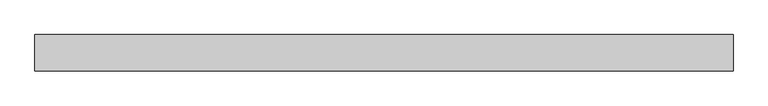
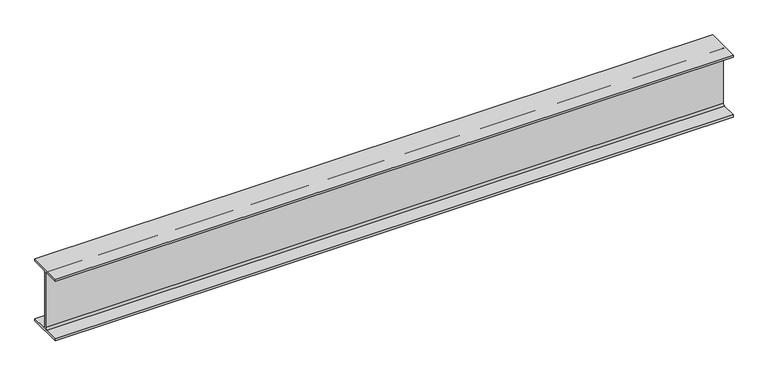
"""IFC4 building model written with IfcOpenShell, lengths in millimetres: beam geometry, Old_Steel Beam_H-KSD3502 : H_SB_ASB_H-250×125x6x9."""

import ifcopenshell
import ifcopenshell.guid

model = None  # the IFC model being written
_history = None  # IfcOwnerHistory: only IFC2X3 demands one
_inside = {}  # id of a spatial element -> (the spatial element, [elements in it])
_under = {}  # id of a project, library or spatial element -> (it, [spatial elements below it])
_declared = {}  # id of a project -> (the project, [libraries it declares])
_typed = {}  # id of a type object -> (the type object, [elements of that type])
_made_of = {}  # id of a material, layer set ... -> (it, [elements and type objects made of it])


def new_model(schema):
    """Start an empty IFC model of exactly this schema.

    Asked for "IFC4X3", IfcOpenShell would pick the latest addendum, in which some entities
    have other attributes; the version numbers below select the first issue.
    IFC2X3 requires an IfcOwnerHistory on every rooted entity: one is made here for all.
    """
    global model, _history
    if schema == "IFC4X3":
        model = ifcopenshell.file(schema_version=(4, 3, 0, 0))
    else:
        model = ifcopenshell.file(schema=schema)
    _inside.clear()
    _under.clear()
    _declared.clear()
    _typed.clear()
    _made_of.clear()
    _history = None
    if model.schema == "IFC2X3":
        org = make("IfcOrganization", Name="unknown")
        user = make(
            "IfcPersonAndOrganization",
            ThePerson=make("IfcPerson", FamilyName="unknown"),
            TheOrganization=org,
        )
        app = make(
            "IfcApplication",
            ApplicationDeveloper=org,
            Version="unknown",
            ApplicationFullName="unknown",
            ApplicationIdentifier="unknown",
        )
        _history = make(
            "IfcOwnerHistory",
            OwningUser=user,
            OwningApplication=app,
            ChangeAction="ADDED",
            CreationDate=0,
        )
    return model


def make(cls, **values):
    """One entity of the class cls with the attributes given. An attribute that is None is left unset."""
    return model.create_entity(
        cls, **{name: value for name, value in values.items() if value is not None}
    )


def rooted(cls, **values):
    """An entity with a GlobalId (a new one), such as an element, a storey or a relation."""
    return make(cls, GlobalId=ifcopenshell.guid.new(), OwnerHistory=_history, **values)


def si_unit(unit_type, name, prefix=None):
    """IfcSIUnit, for example si_unit("LENGTHUNIT", "METRE", prefix="MILLI")."""
    return make("IfcSIUnit", UnitType=unit_type, Prefix=prefix, Name=name)


def assignment(units):
    """IfcUnitAssignment: the units of a project."""
    return None if units is None else make("IfcUnitAssignment", Units=units)


def point(xyz):
    """IfcCartesianPoint."""
    return None if xyz is None else make("IfcCartesianPoint", Coordinates=xyz)


def direction(xyz):
    """IfcDirection."""
    return None if xyz is None else make("IfcDirection", DirectionRatios=xyz)


def frame(location, z_axis=None, x_axis=None):
    """IfcAxis2Placement3D, a coordinate frame: its origin and axes. An axis left out is left unset."""
    return make(
        "IfcAxis2Placement3D",
        Location=point(location),
        Axis=direction(z_axis),
        RefDirection=direction(x_axis),
    )


def frame_2d(location, x_axis=None):
    """IfcAxis2Placement2D, a coordinate frame in the plane: its origin and x axis."""
    return make(
        "IfcAxis2Placement2D", Location=point(location), RefDirection=direction(x_axis)
    )


def origin():
    """The frame at (0, 0, 0) with its axes left unset."""
    return frame((0.0, 0.0, 0.0))


def place(relative_to, where):
    """IfcLocalPlacement: puts the frame where relative to a parent placement (None: the world)."""
    return make(
        "IfcLocalPlacement", PlacementRelTo=relative_to, RelativePlacement=where
    )


def context(
    kind, dimensions, precision=None, world=None, true_north=None, identifier=None
):
    """IfcGeometricRepresentationContext, for example the 3D "Model" context."""
    return make(
        "IfcGeometricRepresentationContext",
        ContextIdentifier=identifier,
        ContextType=kind,
        CoordinateSpaceDimension=dimensions,
        Precision=precision,
        WorldCoordinateSystem=world,
        TrueNorth=true_north,
    )


def project(units=None, contexts=None):
    """IfcProject with its units and contexts."""
    return rooted(
        "IfcProject",
        Name="project",
        RepresentationContexts=contexts,
        UnitsInContext=assignment(units),
    )


def spatial(cls, under=None, at=None, **own):
    """A site, building, storey or space (cls), placed at a placement, below another one or the project."""
    s = rooted(cls, ObjectPlacement=at, **own)
    if under is not None:
        _under.setdefault(under.id(), (under, []))[1].append(s)
    return s


def polyline(points):
    """IfcPolyline through the points."""
    return make("IfcPolyline", Points=[point(p) for p in points])


def circle_curve(where, radius):
    """IfcCircle in the frame where."""
    return make("IfcCircle", Position=where, Radius=radius)


def trimmed(basis, trim1, trim2, sense, master):
    """IfcTrimmedCurve: the piece of a basis curve between two trims."""
    return make(
        "IfcTrimmedCurve",
        BasisCurve=basis,
        Trim1=trim1,
        Trim2=trim2,
        SenseAgreement=sense,
        MasterRepresentation=master,
    )


def segment(curve, same_sense, transition):
    """IfcCompositeCurveSegment."""
    return make(
        "IfcCompositeCurveSegment",
        Transition=transition,
        SameSense=same_sense,
        ParentCurve=curve,
    )


def composite_curve(segments, self_intersect=None):
    """IfcCompositeCurve: segments joined end to end."""
    return make("IfcCompositeCurve", Segments=segments, SelfIntersect=self_intersect)


def outline(outer, holes=None, kind="AREA"):
    """IfcArbitraryClosedProfileDef: a profile drawn as a closed curve; with holes, ...WithVoids."""
    if holes is None:
        return make("IfcArbitraryClosedProfileDef", ProfileType=kind, OuterCurve=outer)
    return make(
        "IfcArbitraryProfileDefWithVoids",
        ProfileType=kind,
        OuterCurve=outer,
        InnerCurves=holes,
    )


def extrude(swept, where, along, depth):
    """IfcExtrudedAreaSolid: the profile swept, set in the frame where, extruded along a direction by depth."""
    return make(
        "IfcExtrudedAreaSolid",
        SweptArea=swept,
        Position=where,
        ExtrudedDirection=direction(along),
        Depth=depth,
    )


def shape(context_of_items, identifier, shape_type, items):
    """IfcShapeRepresentation: the items that make up one representation, for example the "Body"."""
    return make(
        "IfcShapeRepresentation",
        ContextOfItems=context_of_items,
        RepresentationIdentifier=identifier,
        RepresentationType=shape_type,
        Items=items,
    )


def source(mapping_origin, context_of_items, identifier, shape_type, items):
    """IfcRepresentationMap: a shape defined once, which mapped items show again and again."""
    return make(
        "IfcRepresentationMap",
        MappingOrigin=mapping_origin,
        MappedRepresentation=shape(context_of_items, identifier, shape_type, items),
    )


def transform(
    local_origin,
    x_axis=None,
    y_axis=None,
    z_axis=None,
    scale=None,
    scale2=None,
    scale3=None,
    uniform=True,
):
    """IfcCartesianTransformationOperator3D, or its non-uniform kind. x_axis, y_axis, z_axis: its Axis1, 2, 3."""
    if uniform:
        return make(
            "IfcCartesianTransformationOperator3D",
            Axis1=direction(x_axis),
            Axis2=direction(y_axis),
            LocalOrigin=point(local_origin),
            Scale=scale,
            Axis3=direction(z_axis),
        )
    return make(
        "IfcCartesianTransformationOperator3DnonUniform",
        Axis1=direction(x_axis),
        Axis2=direction(y_axis),
        LocalOrigin=point(local_origin),
        Scale=scale,
        Axis3=direction(z_axis),
        Scale2=scale2,
        Scale3=scale3,
    )


def mapped(mapping_source, mapping_target):
    """IfcMappedItem: shows the shape of a source again, moved by a transform."""
    return make(
        "IfcMappedItem", MappingSource=mapping_source, MappingTarget=mapping_target
    )


def made_of(thing, what):
    """Note that an element or type object is made of a material, layer set ...; save() writes the relation."""
    if what is not None:
        _made_of.setdefault(what.id(), (what, []))[1].append(thing)
    return thing


def element(
    cls,
    number,
    at=None,
    inside=None,
    cuts=None,
    type_object=None,
    material=None,
    context=None,
    identifier="Body",
    shape_type=None,
    held_by="IfcProductDefinitionShape",
    body=None,
    shapes=None,
    **own,
):
    """One element of the class cls, such as IfcWall. Its Tag is "e" and its number.

    at: its placement. inside: the storey or other place that contains it. cuts: it is an
    opening in that element (IfcRelVoidsElement). A single representation is given by context,
    identifier, shape_type and body (its items); several are given by shapes. held_by: the class
    of the entity that holds the representations. save() writes the other relations.
    """
    e = rooted(cls, Tag="e%d" % number, ObjectPlacement=at, **own)
    if body is not None:
        shapes = [shape(context, identifier, shape_type, body)]
    if shapes is not None:
        e.Representation = make(held_by, Representations=shapes)
    if inside is not None:
        _inside.setdefault(inside.id(), (inside, []))[1].append(e)
    if cuts is not None:
        rooted(
            "IfcRelVoidsElement", RelatingBuildingElement=cuts, RelatedOpeningElement=e
        )
    if type_object is not None:
        _typed.setdefault(type_object.id(), (type_object, []))[1].append(e)
    return made_of(e, material)


def aggregate(whole, parts):
    """IfcRelAggregates: a whole, such as a stair, and the parts it consists of."""
    return rooted("IfcRelAggregates", RelatingObject=whole, RelatedObjects=parts)


def save(model, path):
    """Write the relations noted so far, then the file.

    IfcRelAggregates (storeys below a building ...), IfcRelContainedInSpatialStructure (elements
    in a storey), IfcRelDefinesByType, IfcRelAssociatesMaterial and IfcRelDeclares: one each for
    every whole, place, type object, material and project.
    """
    for whole, parts in _under.values():
        aggregate(whole, parts)
    for where, things in _inside.values():
        rooted(
            "IfcRelContainedInSpatialStructure",
            RelatedElements=things,
            RelatingStructure=where,
        )
    for kind, things in _typed.values():
        rooted("IfcRelDefinesByType", RelatedObjects=things, RelatingType=kind)
    for what, things in _made_of.values():
        rooted("IfcRelAssociatesMaterial", RelatedObjects=things, RelatingMaterial=what)
    for by, libraries in _declared.values():
        rooted("IfcRelDeclares", RelatingContext=by, RelatedDefinitions=libraries)
    model.write(path)


def beam_56242eb7(model_context):
    return source(origin(), model_context, "Body", "SweptSolid", [
        extrude(outline(composite_curve([segment(polyline([(82.5, -141.5), (82.5, -151.7), (-82.5, -151.7), (-82.5, -141.5), (-11.9, -141.5)]), True, "CONTINUOUS"), segment(trimmed(circle_curve(frame_2d((-11.9, -132.6)), 8.9), [point((-11.9, -141.5))], [point((-3.0, -132.6))], True, "CARTESIAN"), True, "CONTINUOUS"), segment(polyline([(-3.0, -132.6), (-3.0, 132.6)]), True, "CONTINUOUS"), segment(trimmed(circle_curve(frame_2d((-11.9, 132.6)), 8.9), [point((-3.0, 132.6))], [point((-11.9, 141.5))], True, "CARTESIAN"), True, "CONTINUOUS"), segment(polyline([(-11.9, 141.5), (-82.5, 141.5), (-82.5, 151.7), (82.5, 151.7), (82.5, 141.5), (11.9, 141.5)]), True, "CONTINUOUS"), segment(trimmed(circle_curve(frame_2d((11.9, 132.6)), 8.9), [point((11.9, 141.5))], [point((3.0, 132.6))], True, "CARTESIAN"), True, "CONTINUOUS"), segment(polyline([(3.0, 132.6), (3.0, -132.6)]), True, "CONTINUOUS"), segment(trimmed(circle_curve(frame_2d((11.9, -132.6)), 8.9), [point((3.0, -132.6))], [point((11.9, -141.5))], True, "CARTESIAN"), True, "CONTINUOUS"), segment(polyline([(11.9, -141.5), (82.5, -141.5)]), True, "CONTINUOUS")], self_intersect=False)), frame((-1654.8, 0.0, 0.0), z_axis=(1.0, 0.0, 0.0), x_axis=(0.0, 1.0, 0.0)), (0.0, 0.0, 1.0), 3149.3360727),
    ])


if __name__ == "__main__":
    model = new_model("IFC4")
    model_context = context("Model", 3, world=origin())
    ifc_project = project(units=[si_unit("LENGTHUNIT", "METRE", prefix="MILLI")], contexts=[model_context])
    site = spatial("IfcSite", under=ifc_project)
    building = spatial("IfcBuilding", under=site)
    placement = place(None, origin())
    beam_shape = beam_56242eb7(model_context)
    element("IfcBeam", 1, ObjectType="Old_Steel Beam_H-KSD3502 : H_SB_ASB_H-250×125x6x9", at=placement, inside=building, context=model_context, shape_type="MappedRepresentation", body=[
        mapped(beam_shape, transform((0.0, 0.0, 0.0), x_axis=(1.0, 0.0, 0.0), y_axis=(0.0, 1.0, 0.0), z_axis=(0.0, 0.0, 1.0))),
    ])
    save(model, "model.ifc")

# Revit data of these elements
# Type "Old_Steel Beam_H-KSD3502 : H_SB_ASB_H-250×125x6x9"
#   Width = 12.5 cm
#   Web Thickness = 0.6 cm
#   Web Fillet = 1.2 cm
#   Warping Constant = 42539.8 cm⁶
#   Torsional Moment of Inertia = 7.8102 cm⁴
#   Torsional Modulus = 1.0 cm³
#   Section Area = 37.66 cm²
#   Plastic Modulus weak axis = 73.1 cm³
#   Plastic Modulus strong axis = 366.0 cm³
#   Perimeter = 0.97 m²/m
#   Nominal Weight = 29.60 kgf/m
#   Moment of Inertia weak axis = 294.00 cm⁴
#   Moment of Inertia strong axis = 4050.00 cm⁴
#   Height = 25.0 cm
#   Flange Thickness = 0.9 cm
#   Elastic Modulus weak axis = 47.0 cm³
#   Elastic Modulus strong axis = 324.0 cm³
#   Centroid Vertical = 12.5 cm
#   Centroid Horizontal = 6.25 cm
#   Length [instance default] = 1.5240 m
#   Structural Material [instance default] = Steel, 45-345
#   Assembly Code = ""
# Element 1 (IfcBeam, "Old_Steel Beam_H-KSD3502 : H_SB_ASB_H-250×125x6x9")
#   Structural Material = none
# Materials
#   "Steel, 45-345": class "Metal", colour RGB 189 187 185, transparency 0, Description = "Steel 345 MPa", Cost = 0
